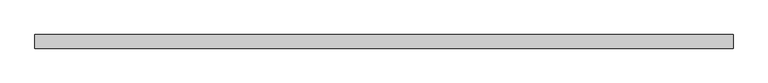
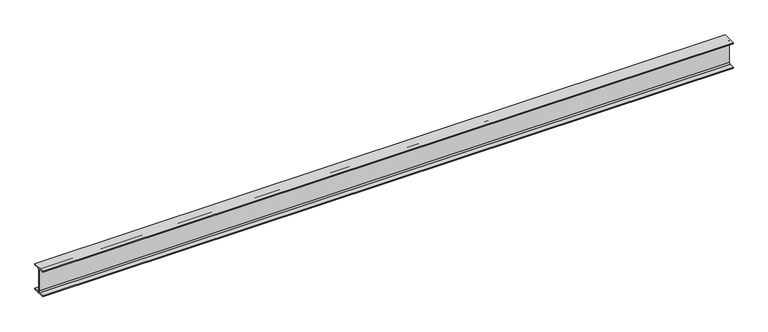
"""IFC4 building model written with IfcOpenShell, lengths in millimetres: beam geometry, 0912_Steel Framing_H-KSD3502 : H_SB_H-200x100x5.5x8."""

from ifc_helpers import new_model, si_unit, point, frame, frame_2d, origin, place, context, project, spatial, polyline, circle_curve, trimmed, segment, composite_curve, outline, extrude, source, transform, mapped, element, save


def beam_dd467f0e(model_context):
    return source(origin(), model_context, "Body", "SweptSolid", [
        extrude(outline(composite_curve([segment(polyline([(50.0, -92.0), (50.0, -100.0), (-50.0, -100.0), (-50.0, -92.0), (-13.75, -92.0)]), True, "CONTINUOUS"), segment(trimmed(circle_curve(frame_2d((-13.75, -81.0)), 11.0), [point((-13.75, -92.0))], [point((-2.75, -81.0))], True, "CARTESIAN"), True, "CONTINUOUS"), segment(polyline([(-2.75, -81.0), (-2.75, 81.0)]), True, "CONTINUOUS"), segment(trimmed(circle_curve(frame_2d((-13.75, 81.0)), 11.0), [point((-2.75, 81.0))], [point((-13.75, 92.0))], True, "CARTESIAN"), True, "CONTINUOUS"), segment(polyline([(-13.75, 92.0), (-50.0, 92.0), (-50.0, 100.0), (50.0, 100.0), (50.0, 92.0), (13.75, 92.0)]), True, "CONTINUOUS"), segment(trimmed(circle_curve(frame_2d((13.75, 81.0)), 11.0), [point((13.75, 92.0))], [point((2.75, 81.0))], True, "CARTESIAN"), True, "CONTINUOUS"), segment(polyline([(2.75, 81.0), (2.75, -81.0)]), True, "CONTINUOUS"), segment(trimmed(circle_curve(frame_2d((13.75, -81.0)), 11.0), [point((2.75, -81.0))], [point((13.75, -92.0))], True, "CARTESIAN"), True, "CONTINUOUS"), segment(polyline([(13.75, -92.0), (50.0, -92.0)]), True, "CONTINUOUS")], self_intersect=False)), frame((-2509.476368, 0.0, 0.0), z_axis=(1.0, 0.0, 0.0), x_axis=(0.0, 1.0, 0.0)), (0.0, 0.0, 1.0), 5119.4514916),
    ])


if __name__ == "__main__":
    model = new_model("IFC4")
    model_context = context("Model", 3, world=origin())
    ifc_project = project(units=[si_unit("LENGTHUNIT", "METRE", prefix="MILLI")], contexts=[model_context])
    site = spatial("IfcSite", under=ifc_project)
    building = spatial("IfcBuilding", under=site)
    placement = place(None, origin())
    beam_shape = beam_dd467f0e(model_context)
    element("IfcBeam", 1, ObjectType="0912_Steel Framing_H-KSD3502 : H_SB_H-200x100x5.5x8", at=placement, inside=building, context=model_context, shape_type="MappedRepresentation", body=[
        mapped(beam_shape, transform((0.0, 0.0, 0.0), x_axis=(1.0, 0.0, 0.0), y_axis=(0.0, 1.0, 0.0), z_axis=(0.0, 0.0, 1.0))),
    ])
    save(model, "model.ifc")

# Revit data of these elements
# Type "0912_Steel Framing_H-KSD3502 : H_SB_H-200x100x5.5x8"
#   Width = 10.0 cm
#   Web Thickness = 0.55 cm
#   Web Fillet = 1.1 cm
#   Warping Constant = 12288.0 cm⁶
#   W = 0
#   Torsional Moment of Inertia = 4.4781 cm⁴
#   Section Area = 27.16 cm²
#   Plastic Modulus weak axis = 41.9 cm³
#   Plastic Modulus strong axis = 209.0 cm³
#   Perimeter = 0.77 m²/m
#   Nominal Weight = 21.30 kgf/m
#   Moment of Inertia weak axis = 134.00 cm⁴
#   Moment of Inertia strong axis = 1840.00 cm⁴
#   Height = 20.0 cm
#   Flange Thickness = 0.8 cm
#   Elastic Modulus weak axis = 26.8 cm³
#   Elastic Modulus strong axis = 184.0 cm³
#   Centroid Vertical = 10.0 cm
#   Centroid Horizontal = 5.0 cm
#   Ix = 18400000
#   Length [instance default] = 1524 mm
#   Zx = 209000
#   b = 100 mm
#   h = 200 mm
#   r = 11 mm
#   s = 5.5 mm
#   t = 8 mm
#   A = 0.002716 m²
#   Structural Material [instance default] = Steel, 45-345
#   Assembly Code = ""
# Element 1 (IfcBeam, "0912_Steel Framing_H-KSD3502 : H_SB_H-200x100x5.5x8")
#   Materials on its faces: "Steel, 45-345"
# Materials
#   "Steel, 45-345": class "Metal", colour RGB 189 187 185, transparency 0, Description = "Steel 345 MPa", Cost = 0
